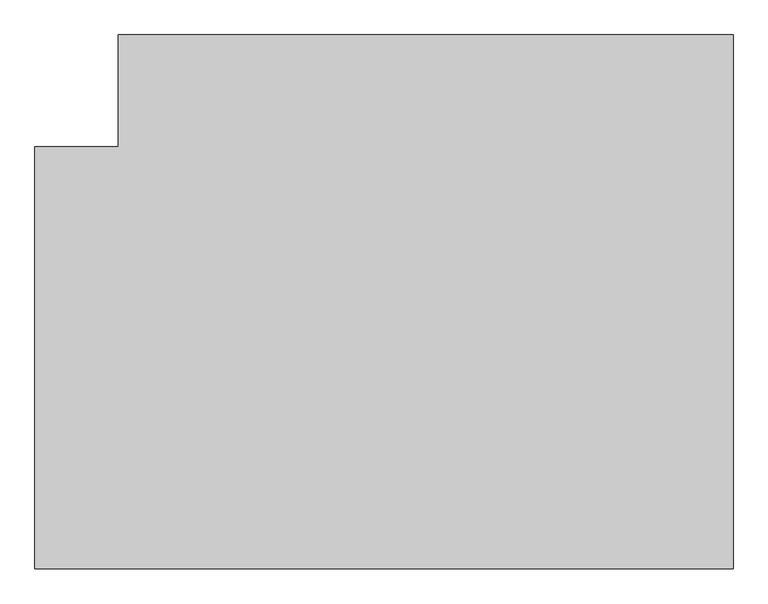
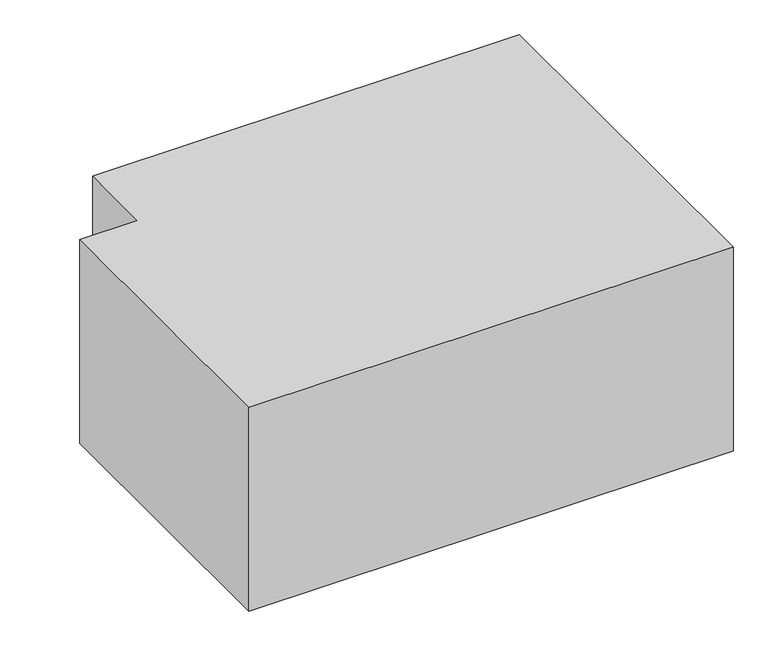
"""IFC4 building model written with IfcOpenShell, lengths in millimetres: proxy geometry, 0_3d."""

from ifc_helpers import new_model, si_unit, origin, origin_with_axes, place, context, project, spatial, polyline, outline, extrude, source, transform, mapped, element, save


def generic_models_219b7667(model_context):
    return source(origin(), model_context, "Body", "SweptSolid", [
        extrude(outline(polyline([(670.0, 4297.8619019), (5620.0, 4297.8619019), (5620.0, 0.0), (0.0, 0.0), (0.0, 3397.8619019), (670.0, 3397.8619019), (670.0, 4297.8619019)])), origin_with_axes(), (0.0, 0.0, 1.0), 2500.0),
    ])


if __name__ == "__main__":
    model = new_model("IFC4")
    model_context = context("Model", 3, world=origin())
    ifc_project = project(units=[si_unit("LENGTHUNIT", "METRE", prefix="MILLI")], contexts=[model_context])
    site = spatial("IfcSite", under=ifc_project)
    building = spatial("IfcBuilding", under=site)
    placement = place(None, origin())
    generic_models_shape = generic_models_219b7667(model_context)
    element("IfcBuildingElementProxy", 1, Name="0_3d", ObjectType="0_3d", at=placement, inside=building, context=model_context, shape_type="MappedRepresentation", body=[
        mapped(generic_models_shape, transform((0.0, 0.0, 0.0), x_axis=(1.0, 0.0, 0.0), y_axis=(0.0, 1.0, 0.0), z_axis=(0.0, 0.0, 1.0))),
    ])
    save(model, "model.ifc")

# Revit data of these elements
# Element 1 (IfcBuildingElementProxy, "0_3d")
#   Materials on its faces: "*1"
# Materials
#   "*1": class "Unassigned", colour RGB 175 175 175, transparency 0
